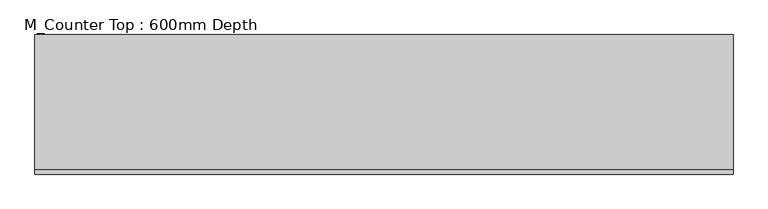
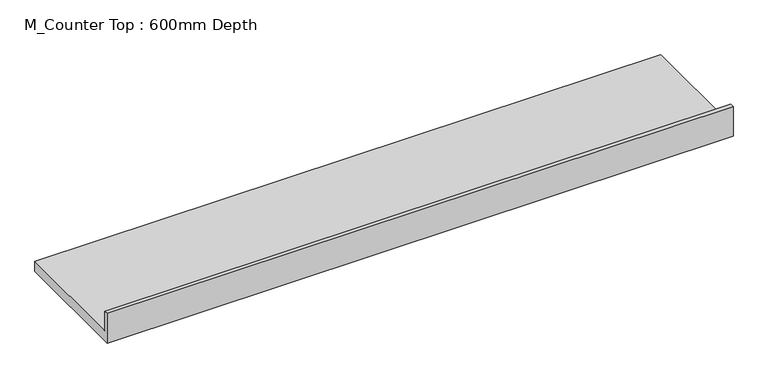
"""IFC4 building model written with IfcOpenShell, lengths in millimetres: furniture geometry, M_Counter Top : 600mm Depth."""

from ifc_helpers import new_model, si_unit, frame, origin, place, context, project, spatial, polyline, outline, extrude, source, transform, mapped, element, save


def m_counter_top_600mm_depth_e6b45aca(model_context):
    return source(origin(), model_context, "Body", "SweptSolid", [
        extrude(outline(polyline([(0.0, 1016.0), (19.05, 1016.0), (19.05, 914.4), (609.6, 914.4), (609.6, 863.6), (0.0, 863.6), (0.0, 1016.0)])), frame((-1200.4622951, 0.0, 0.0), z_axis=(1.0, 0.0, 0.0), x_axis=(0.0, 1.0, 0.0)), (0.0, 0.0, 1.0), 3048.0),
    ])


if __name__ == "__main__":
    model = new_model("IFC4")
    model_context = context("Model", 3, world=origin())
    ifc_project = project(units=[si_unit("LENGTHUNIT", "METRE", prefix="MILLI")], contexts=[model_context])
    site = spatial("IfcSite", under=ifc_project)
    building = spatial("IfcBuilding", under=site)
    placement = place(None, origin())
    m_counter_top_600mm_depth_shape = m_counter_top_600mm_depth_e6b45aca(model_context)
    element("IfcFurniture", 1, ObjectType="M_Counter Top : 600mm Depth", at=placement, inside=building, context=model_context, shape_type="MappedRepresentation", body=[
        mapped(m_counter_top_600mm_depth_shape, transform((0.0, 0.0, 0.0), x_axis=(1.0, 0.0, 0.0), y_axis=(0.0, 1.0, 0.0), z_axis=(0.0, 0.0, 1.0))),
    ])
    save(model, "model.ifc")

# Revit data of these elements
# Type "M_Counter Top : 600mm Depth"
#   Counter Thickness = 0' - 2"
#   Depth = 2' - 0"
#   Height = 3' - 0"
#   Length [instance default] = 8' - 2.4252"
#   Counter Top Material = none
# Element 1 (IfcFurniture, "M_Counter Top : 600mm Depth")
#   Length = 10' - 0"
#   Materials on its faces: "Counter Top"
# Materials
#   "Counter Top": class "Wood", colour RGB 226 177 128, transparency 0
